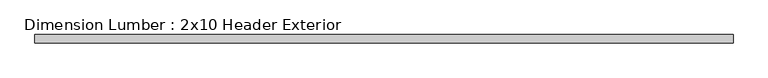
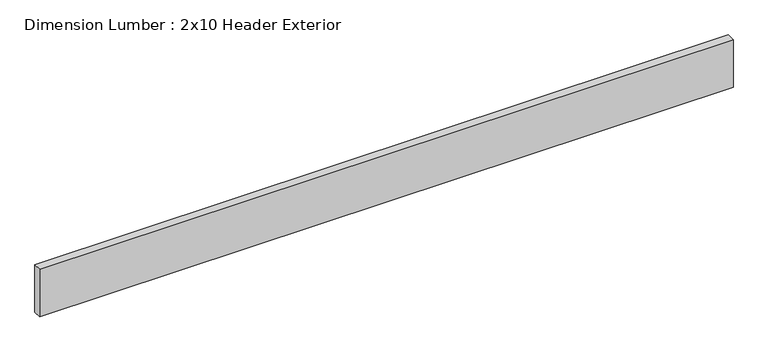
"""IFC4 building model written with IfcOpenShell, lengths in millimetres: beam geometry, Dimension Lumber : 2x10 Header Exterior."""

from ifc_helpers import new_model, si_unit, frame, origin, place, context, project, spatial, polyline, outline, extrude, source, transform, mapped, element, save


def dimension_lumber_2x10_header_exterior_df58e940(model_context):
    return source(origin(), model_context, "Body", "SweptSolid", [
        extrude(outline(polyline([(1646.2375, 19.05), (1646.2375, -19.05), (-1592.2625, -19.05), (-1592.2625, 19.05), (1646.2375, 19.05)])), frame((0.0, 0.0, -117.475), z_axis=(0.0, 0.0, 1.0), x_axis=(1.0, 0.0, 0.0)), (0.0, 0.0, 1.0), 234.95),
    ])


if __name__ == "__main__":
    model = new_model("IFC4")
    model_context = context("Model", 3, world=origin())
    ifc_project = project(units=[si_unit("LENGTHUNIT", "METRE", prefix="MILLI")], contexts=[model_context])
    site = spatial("IfcSite", under=ifc_project)
    building = spatial("IfcBuilding", under=site)
    placement = place(None, origin())
    dimension_lumber_2x10_header_exterior_shape = dimension_lumber_2x10_header_exterior_df58e940(model_context)
    element("IfcBeam", 1, ObjectType="Dimension Lumber : 2x10 Header Exterior", at=placement, inside=building, context=model_context, shape_type="MappedRepresentation", body=[
        mapped(dimension_lumber_2x10_header_exterior_shape, transform((0.0, 0.0, 0.0), x_axis=(1.0, 0.0, 0.0), y_axis=(0.0, 1.0, 0.0), z_axis=(0.0, 0.0, 1.0))),
    ])
    save(model, "model.ifc")

# Revit data of these elements
# Type "Dimension Lumber : 2x10 Header Exterior"
#   Assembly Code = "B10"
#   A = 0.0963889 SF
#   Length [instance default] = 5' - 0"
#   b = 0' - 1 1/2"
#   d = 0' - 9 1/4"
#   Structural Material [instance default] = Softwood, Lumber
# Element 1 (IfcBeam, "Dimension Lumber : 2x10 Header Exterior")
#   Structural Material = Douglas Fir #2
#   Materials on its faces: "Douglas Fir #2"
# Materials
#   "Softwood, Lumber": class "Wood", colour RGB 223 192 134, transparency 0, Description = "Pinus Echinata", Cost = 0
#   "Douglas Fir #2": class "Wood", colour RGB 223 192 134, transparency 0, Description = "Pinus Echinata", Cost = 0
